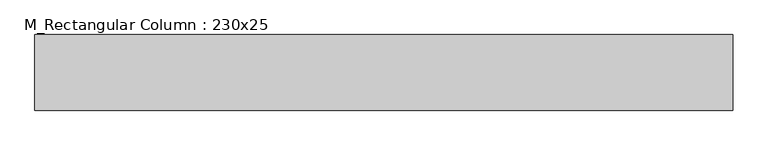
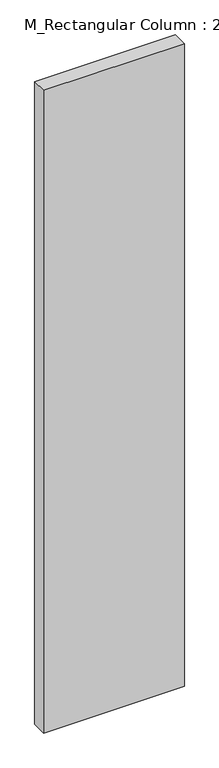
"""IFC4 building model written with IfcOpenShell, lengths in millimetres: column geometry, M_Rectangular Column : 230x25."""

from ifc_helpers import new_model, si_unit, frame, origin, place, context, project, spatial, polyline, outline, extrude, source, transform, mapped, element, save


def m_rectangular_column_230x25_da6e8c6c(model_context):
    return source(origin(), model_context, "Body", "SweptSolid", [
        extrude(outline(polyline([(1150.0, 125.0), (1150.0, -125.0), (-1150.0, -125.0), (-1150.0, 125.0), (1150.0, 125.0)])), frame((0.0, 0.0, -3200.0), z_axis=(0.0, 0.0, 1.0), x_axis=(1.0, 0.0, 0.0)), (0.0, 0.0, 1.0), 11100.0),
    ])


if __name__ == "__main__":
    model = new_model("IFC4")
    model_context = context("Model", 3, world=origin())
    ifc_project = project(units=[si_unit("LENGTHUNIT", "METRE", prefix="MILLI")], contexts=[model_context])
    site = spatial("IfcSite", under=ifc_project)
    building = spatial("IfcBuilding", under=site)
    placement = place(None, origin())
    m_rectangular_column_230x25_shape = m_rectangular_column_230x25_da6e8c6c(model_context)
    element("IfcColumn", 1, ObjectType="M_Rectangular Column : 230x25", at=placement, inside=building, context=model_context, shape_type="MappedRepresentation", body=[
        mapped(m_rectangular_column_230x25_shape, transform((0.0, 0.0, 0.0), x_axis=(1.0, 0.0, 0.0), y_axis=(0.0, 1.0, 0.0), z_axis=(0.0, 0.0, 1.0))),
    ])
    save(model, "model.ifc")

# Revit data of these elements
# Type "M_Rectangular Column : 230x25"
#   Depth = 25 cm
#   Offset Base = 0 cm
#   Offset Top = 0 cm
#   Width = 230 cm
#   Material = none
